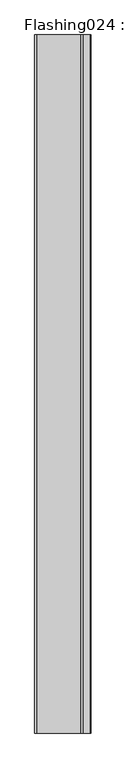
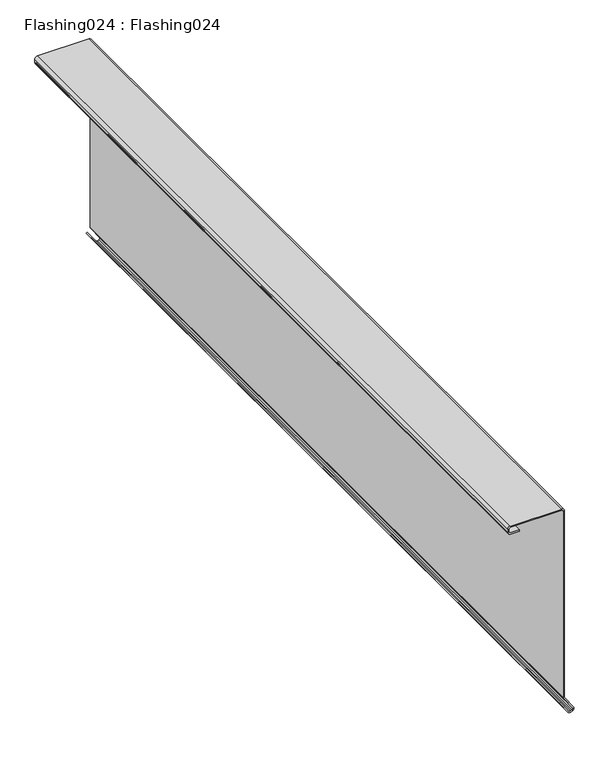
"""IFC4 building model written with IfcOpenShell, lengths in millimetres: proxy geometry, Flashing024 : Flashing024."""

from ifc_helpers import new_model, si_unit, point, frame, frame_2d, origin, place, context, project, spatial, polyline, circle_curve, trimmed, segment, composite_curve, outline, extrude, source, transform, mapped, element, save


def flashing024_flashing024_9ad17ddb(model_context):
    return source(origin(), model_context, "Body", "SweptSolid", [
        extrude(outline(composite_curve([segment(trimmed(circle_curve(frame_2d((41323.8783762, 6183.9556944)), 6.35), [point((41320.2092308, 6178.7730434))], [point((41318.4012804, 6187.1687804))], False, "CARTESIAN"), True, "CONTINUOUS"), segment(polyline([(41318.4012804, 6187.1687804), (41320.1425067, 6190.1369125)]), True, "CONTINUOUS"), segment(trimmed(circle_curve(frame_2d((41325.6196026, 6186.9238265)), 6.35), [point((41320.1425067, 6190.1369125))], [point((41329.2370767, 6192.1426751))], False, "CARTESIAN"), True, "CONTINUOUS"), segment(polyline([(41329.2370767, 6192.1426751), (41359.2301171, 6171.3528311)]), True, "CONTINUOUS"), segment(trimmed(circle_curve(frame_2d((41362.8475913, 6176.5716797)), 6.35), [point((41359.2301171, 6171.3528311))], [point((41362.8475913, 6170.2216797))], True, "CARTESIAN"), True, "CONTINUOUS"), segment(polyline([(41362.8475913, 6170.2216797), (41842.9189039, 6170.2216797)]), True, "CONTINUOUS"), segment(trimmed(circle_curve(frame_2d((41842.9189039, 6163.8716797)), 6.35), [point((41842.9189039, 6170.2216797))], [point((41849.2689039, 6163.8716797))], False, "CARTESIAN"), True, "CONTINUOUS"), segment(polyline([(41849.2689039, 6163.8716797), (41849.2689039, 6038.1540605)]), True, "CONTINUOUS"), segment(trimmed(circle_curve(frame_2d((41842.9189039, 6038.1540605)), 6.35), [point((41849.2689039, 6038.1540605))], [point((41842.9189039, 6031.8040605))], False, "CARTESIAN"), True, "CONTINUOUS"), segment(polyline([(41842.9189039, 6031.8040605), (41835.0524976, 6031.8040605)]), True, "CONTINUOUS"), segment(trimmed(circle_curve(frame_2d((41835.0524976, 6038.1540605)), 6.35), [point((41835.0524976, 6031.8040605))], [point((41828.7024976, 6038.1540605))], False, "CARTESIAN"), True, "CONTINUOUS"), segment(polyline([(41828.7024976, 6038.1540605), (41828.7024976, 6060.1805253), (41831.7024976, 6060.1805253), (41831.7024976, 6038.1540605)]), True, "CONTINUOUS"), segment(trimmed(circle_curve(frame_2d((41835.0524976, 6038.1540605)), 3.35), [point((41831.7024976, 6038.1540605))], [point((41835.0524976, 6034.8040605))], True, "CARTESIAN"), True, "CONTINUOUS"), segment(polyline([(41835.0524976, 6034.8040605), (41842.9189039, 6034.8040605)]), True, "CONTINUOUS"), segment(trimmed(circle_curve(frame_2d((41842.9189039, 6038.1540605)), 3.35), [point((41842.9189039, 6034.8040605))], [point((41846.2689039, 6038.1540605))], True, "CARTESIAN"), True, "CONTINUOUS"), segment(polyline([(41846.2689039, 6038.1540605), (41846.2689039, 6163.8716797)]), True, "CONTINUOUS"), segment(trimmed(circle_curve(frame_2d((41842.9189039, 6163.8716797)), 3.35), [point((41846.2689039, 6163.8716797))], [point((41842.9189039, 6167.2216797))], True, "CARTESIAN"), True, "CONTINUOUS"), segment(polyline([(41842.9189039, 6167.2216797), (41362.8475913, 6167.2216797)]), True, "CONTINUOUS"), segment(trimmed(circle_curve(frame_2d((41362.8475913, 6176.5716797)), 9.35), [point((41362.8475913, 6167.2216797))], [point((41357.5210742, 6168.8872333))], False, "CARTESIAN"), True, "CONTINUOUS"), segment(polyline([(41357.5210742, 6168.8872333), (41327.5280338, 6189.6770774)]), True, "CONTINUOUS"), segment(trimmed(circle_curve(frame_2d((41325.6196026, 6186.9238265)), 3.35), [point((41327.5280338, 6189.6770774))], [point((41322.730111, 6188.6189191))], True, "CARTESIAN"), True, "CONTINUOUS"), segment(polyline([(41322.730111, 6188.6189191), (41320.9888847, 6185.650787)]), True, "CONTINUOUS"), segment(trimmed(circle_curve(frame_2d((41323.8783762, 6183.9556944)), 3.35), [point((41320.9888847, 6185.650787))], [point((41321.9426853, 6181.2215399))], True, "CARTESIAN"), True, "CONTINUOUS"), segment(polyline([(41321.9426853, 6181.2215399), (41352.3883692, 6159.6670035), (41350.6549147, 6157.218507), (41320.2092308, 6178.7730434)]), True, "CONTINUOUS")], self_intersect=False)), frame((0.0, 2217.3609988, 0.0), z_axis=(0.0, 1.0, 0.0), x_axis=(0.0, 0.0, 1.0)), (0.0, 0.0, 1.0), 2000.0),
    ])


if __name__ == "__main__":
    model = new_model("IFC4")
    model_context = context("Model", 3, world=origin())
    ifc_project = project(units=[si_unit("LENGTHUNIT", "METRE", prefix="MILLI")], contexts=[model_context])
    site = spatial("IfcSite", under=ifc_project)
    building = spatial("IfcBuilding", under=site)
    placement = place(None, origin())
    flashing024_flashing024_shape = flashing024_flashing024_9ad17ddb(model_context)
    element("IfcBuildingElementProxy", 1, Name="Flashing024 : Flashing024", ObjectType="Flashing024 : Flashing024", at=placement, inside=building, context=model_context, shape_type="MappedRepresentation", body=[
        mapped(flashing024_flashing024_shape, transform((0.0, 0.0, 0.0), x_axis=(1.0, 0.0, 0.0), y_axis=(0.0, 1.0, 0.0), z_axis=(0.0, 0.0, 1.0))),
    ])
    save(model, "model.ifc")

# Revit data of these elements
# Type "Flashing024 : Flashing024"
#   NameOverride = "Flashing024"
# Element 1 (IfcBuildingElementProxy, "Flashing024 : Flashing024")
#   Materials on its faces: "BRAKE METAL EAVE TRIM TO MATCH STANDING SEAM COLOR"
# Materials
#   "BRAKE METAL EAVE TRIM TO MATCH STANDING SEAM COLOR": class "Unassigned", colour RGB 128 128 128, transparency 0, Cost = 0
